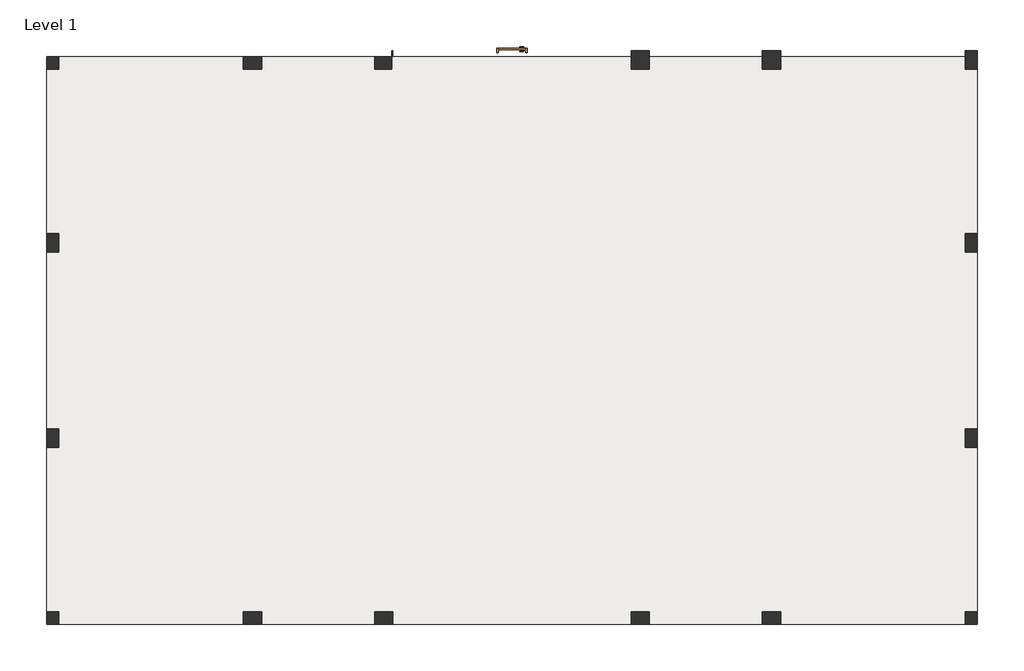
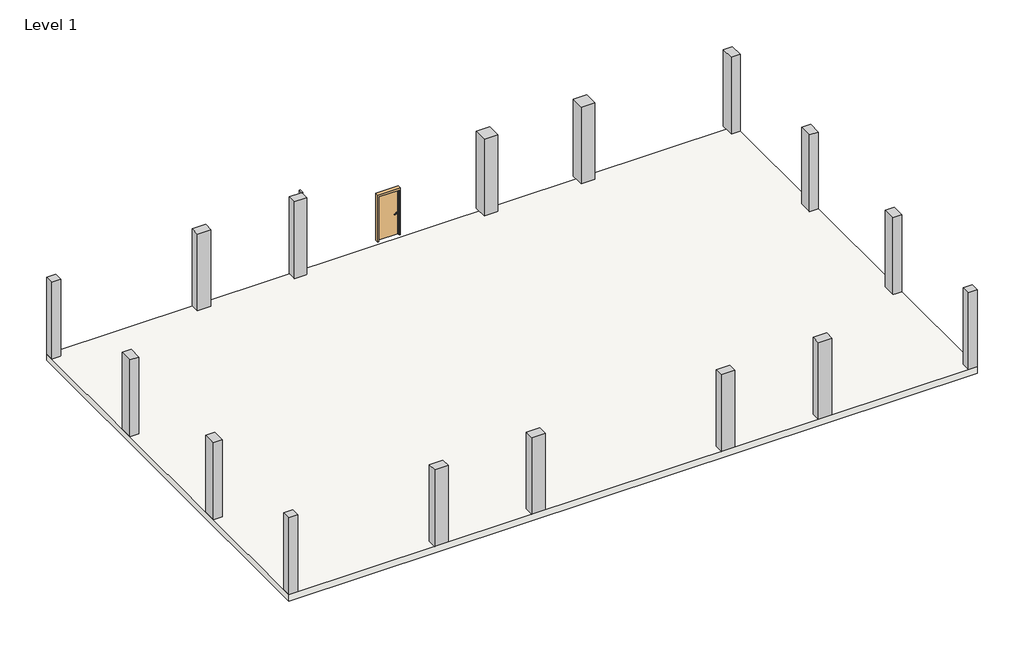
# One storey: 16 columns, 1 door, 1 slab.
"""IFC4 building model written with IfcOpenShell, lengths in millimetres."""

import ifcopenshell
import ifcopenshell.guid

model = None  # the IFC model being written
_history = None  # IfcOwnerHistory: only IFC2X3 demands one
_inside = {}  # id of a spatial element -> (the spatial element, [elements in it])
_under = {}  # id of a project, library or spatial element -> (it, [spatial elements below it])
_declared = {}  # id of a project -> (the project, [libraries it declares])
_typed = {}  # id of a type object -> (the type object, [elements of that type])
_made_of = {}  # id of a material, layer set ... -> (it, [elements and type objects made of it])


def new_model(schema):
    """Start an empty IFC model of exactly this schema.

    Asked for "IFC4X3", IfcOpenShell would pick the latest addendum, in which some entities
    have other attributes; the version numbers below select the first issue.
    IFC2X3 requires an IfcOwnerHistory on every rooted entity: one is made here for all.
    """
    global model, _history
    if schema == "IFC4X3":
        model = ifcopenshell.file(schema_version=(4, 3, 0, 0))
    else:
        model = ifcopenshell.file(schema=schema)
    _inside.clear()
    _under.clear()
    _declared.clear()
    _typed.clear()
    _made_of.clear()
    _history = None
    if model.schema == "IFC2X3":
        org = make("IfcOrganization", Name="unknown")
        user = make(
            "IfcPersonAndOrganization",
            ThePerson=make("IfcPerson", FamilyName="unknown"),
            TheOrganization=org,
        )
        app = make(
            "IfcApplication",
            ApplicationDeveloper=org,
            Version="unknown",
            ApplicationFullName="unknown",
            ApplicationIdentifier="unknown",
        )
        _history = make(
            "IfcOwnerHistory",
            OwningUser=user,
            OwningApplication=app,
            ChangeAction="ADDED",
            CreationDate=0,
        )
    return model


def make(cls, **values):
    """One entity of the class cls with the attributes given. An attribute that is None is left unset."""
    return model.create_entity(
        cls, **{name: value for name, value in values.items() if value is not None}
    )


def rooted(cls, **values):
    """An entity with a GlobalId (a new one), such as an element, a storey or a relation."""
    return make(cls, GlobalId=ifcopenshell.guid.new(), OwnerHistory=_history, **values)


def si_unit(unit_type, name, prefix=None):
    """IfcSIUnit, for example si_unit("LENGTHUNIT", "METRE", prefix="MILLI")."""
    return make("IfcSIUnit", UnitType=unit_type, Prefix=prefix, Name=name)


def assignment(units):
    """IfcUnitAssignment: the units of a project."""
    return None if units is None else make("IfcUnitAssignment", Units=units)


def point(xyz):
    """IfcCartesianPoint."""
    return None if xyz is None else make("IfcCartesianPoint", Coordinates=xyz)


def direction(xyz):
    """IfcDirection."""
    return None if xyz is None else make("IfcDirection", DirectionRatios=xyz)


def frame(location, z_axis=None, x_axis=None):
    """IfcAxis2Placement3D, a coordinate frame: its origin and axes. An axis left out is left unset."""
    return make(
        "IfcAxis2Placement3D",
        Location=point(location),
        Axis=direction(z_axis),
        RefDirection=direction(x_axis),
    )


def frame_2d(location, x_axis=None):
    """IfcAxis2Placement2D, a coordinate frame in the plane: its origin and x axis."""
    return make(
        "IfcAxis2Placement2D", Location=point(location), RefDirection=direction(x_axis)
    )


def origin():
    """The frame at (0, 0, 0) with its axes left unset."""
    return frame((0.0, 0.0, 0.0))


def origin_with_axes():
    """The frame at (0, 0, 0) with the z axis (0, 0, 1) and the x axis (1, 0, 0) written out."""
    return frame((0.0, 0.0, 0.0), z_axis=(0.0, 0.0, 1.0), x_axis=(1.0, 0.0, 0.0))


def place(relative_to, where):
    """IfcLocalPlacement: puts the frame where relative to a parent placement (None: the world)."""
    return make(
        "IfcLocalPlacement", PlacementRelTo=relative_to, RelativePlacement=where
    )


def context(
    kind, dimensions, precision=None, world=None, true_north=None, identifier=None
):
    """IfcGeometricRepresentationContext, for example the 3D "Model" context."""
    return make(
        "IfcGeometricRepresentationContext",
        ContextIdentifier=identifier,
        ContextType=kind,
        CoordinateSpaceDimension=dimensions,
        Precision=precision,
        WorldCoordinateSystem=world,
        TrueNorth=true_north,
    )


def project(units=None, contexts=None):
    """IfcProject with its units and contexts."""
    return rooted(
        "IfcProject",
        Name="project",
        RepresentationContexts=contexts,
        UnitsInContext=assignment(units),
    )


def spatial(cls, under=None, at=None, **own):
    """A site, building, storey or space (cls), placed at a placement, below another one or the project."""
    s = rooted(cls, ObjectPlacement=at, **own)
    if under is not None:
        _under.setdefault(under.id(), (under, []))[1].append(s)
    return s


def polyline(points):
    """IfcPolyline through the points."""
    return make("IfcPolyline", Points=[point(p) for p in points])


def circle_curve(where, radius):
    """IfcCircle in the frame where."""
    return make("IfcCircle", Position=where, Radius=radius)


def ellipse_curve(where, semi_axis1, semi_axis2):
    """IfcEllipse in the frame where."""
    return make(
        "IfcEllipse", Position=where, SemiAxis1=semi_axis1, SemiAxis2=semi_axis2
    )


def trimmed(basis, trim1, trim2, sense, master):
    """IfcTrimmedCurve: the piece of a basis curve between two trims."""
    return make(
        "IfcTrimmedCurve",
        BasisCurve=basis,
        Trim1=trim1,
        Trim2=trim2,
        SenseAgreement=sense,
        MasterRepresentation=master,
    )


def segment(curve, same_sense, transition):
    """IfcCompositeCurveSegment."""
    return make(
        "IfcCompositeCurveSegment",
        Transition=transition,
        SameSense=same_sense,
        ParentCurve=curve,
    )


def composite_curve(segments, self_intersect=None):
    """IfcCompositeCurve: segments joined end to end."""
    return make("IfcCompositeCurve", Segments=segments, SelfIntersect=self_intersect)


def outline(outer, holes=None, kind="AREA"):
    """IfcArbitraryClosedProfileDef: a profile drawn as a closed curve; with holes, ...WithVoids."""
    if holes is None:
        return make("IfcArbitraryClosedProfileDef", ProfileType=kind, OuterCurve=outer)
    return make(
        "IfcArbitraryProfileDefWithVoids",
        ProfileType=kind,
        OuterCurve=outer,
        InnerCurves=holes,
    )


def extrude(swept, where, along, depth):
    """IfcExtrudedAreaSolid: the profile swept, set in the frame where, extruded along a direction by depth."""
    return make(
        "IfcExtrudedAreaSolid",
        SweptArea=swept,
        Position=where,
        ExtrudedDirection=direction(along),
        Depth=depth,
    )


def faces_of(points, faces, orient=None, outer=None):
    """IfcFace entities. A face is a list of loops; a loop is a list of indices into points, from 0.

    orient and outer hold one flag for each loop. By default every Orientation is true, the
    first loop of a face is its IfcFaceOuterBound and the others are IfcFaceBound.
    """
    made = []
    for i, loops in enumerate(faces):
        bounds = []
        for j, loop in enumerate(loops):
            is_outer = j == 0 if outer is None else outer[i][j]
            bounds.append(
                make(
                    "IfcFaceOuterBound" if is_outer else "IfcFaceBound",
                    Bound=make("IfcPolyLoop", Polygon=[points[k] for k in loop]),
                    Orientation=True if orient is None else orient[i][j],
                )
            )
        made.append(make("IfcFace", Bounds=bounds))
    return made


def faceted_brep(points, faces, orient=None, outer=None, voids=None):
    """IfcFacetedBrep: a solid bounded by flat faces; with voids (closed shells), ...WithVoids."""
    shared = [point(p) for p in points]
    hull = make("IfcClosedShell", CfsFaces=faces_of(shared, faces, orient, outer))
    if voids is None:
        return make("IfcFacetedBrep", Outer=hull)
    return make(
        "IfcFacetedBrepWithVoids",
        Outer=hull,
        Voids=[
            make(cls, CfsFaces=faces_of(shared, fs, o, b)) for cls, fs, o, b in voids
        ],
    )


def shape(context_of_items, identifier, shape_type, items):
    """IfcShapeRepresentation: the items that make up one representation, for example the "Body"."""
    return make(
        "IfcShapeRepresentation",
        ContextOfItems=context_of_items,
        RepresentationIdentifier=identifier,
        RepresentationType=shape_type,
        Items=items,
    )


def source(mapping_origin, context_of_items, identifier, shape_type, items):
    """IfcRepresentationMap: a shape defined once, which mapped items show again and again."""
    return make(
        "IfcRepresentationMap",
        MappingOrigin=mapping_origin,
        MappedRepresentation=shape(context_of_items, identifier, shape_type, items),
    )


def transform(
    local_origin,
    x_axis=None,
    y_axis=None,
    z_axis=None,
    scale=None,
    scale2=None,
    scale3=None,
    uniform=True,
):
    """IfcCartesianTransformationOperator3D, or its non-uniform kind. x_axis, y_axis, z_axis: its Axis1, 2, 3."""
    if uniform:
        return make(
            "IfcCartesianTransformationOperator3D",
            Axis1=direction(x_axis),
            Axis2=direction(y_axis),
            LocalOrigin=point(local_origin),
            Scale=scale,
            Axis3=direction(z_axis),
        )
    return make(
        "IfcCartesianTransformationOperator3DnonUniform",
        Axis1=direction(x_axis),
        Axis2=direction(y_axis),
        LocalOrigin=point(local_origin),
        Scale=scale,
        Axis3=direction(z_axis),
        Scale2=scale2,
        Scale3=scale3,
    )


def mapped(mapping_source, mapping_target):
    """IfcMappedItem: shows the shape of a source again, moved by a transform."""
    return make(
        "IfcMappedItem", MappingSource=mapping_source, MappingTarget=mapping_target
    )


def made_of(thing, what):
    """Note that an element or type object is made of a material, layer set ...; save() writes the relation."""
    if what is not None:
        _made_of.setdefault(what.id(), (what, []))[1].append(thing)
    return thing


def element(
    cls,
    number,
    at=None,
    inside=None,
    cuts=None,
    type_object=None,
    material=None,
    context=None,
    identifier="Body",
    shape_type=None,
    held_by="IfcProductDefinitionShape",
    body=None,
    shapes=None,
    **own,
):
    """One element of the class cls, such as IfcWall. Its Tag is "e" and its number.

    at: its placement. inside: the storey or other place that contains it. cuts: it is an
    opening in that element (IfcRelVoidsElement). A single representation is given by context,
    identifier, shape_type and body (its items); several are given by shapes. held_by: the class
    of the entity that holds the representations. save() writes the other relations.
    """
    e = rooted(cls, Tag="e%d" % number, ObjectPlacement=at, **own)
    if body is not None:
        shapes = [shape(context, identifier, shape_type, body)]
    if shapes is not None:
        e.Representation = make(held_by, Representations=shapes)
    if inside is not None:
        _inside.setdefault(inside.id(), (inside, []))[1].append(e)
    if cuts is not None:
        rooted(
            "IfcRelVoidsElement", RelatingBuildingElement=cuts, RelatedOpeningElement=e
        )
    if type_object is not None:
        _typed.setdefault(type_object.id(), (type_object, []))[1].append(e)
    return made_of(e, material)


def aggregate(whole, parts):
    """IfcRelAggregates: a whole, such as a stair, and the parts it consists of."""
    return rooted("IfcRelAggregates", RelatingObject=whole, RelatedObjects=parts)


def save(model, path):
    """Write the relations noted so far, then the file.

    IfcRelAggregates (storeys below a building ...), IfcRelContainedInSpatialStructure (elements
    in a storey), IfcRelDefinesByType, IfcRelAssociatesMaterial and IfcRelDeclares: one each for
    every whole, place, type object, material and project.
    """
    for whole, parts in _under.values():
        aggregate(whole, parts)
    for where, things in _inside.values():
        rooted(
            "IfcRelContainedInSpatialStructure",
            RelatedElements=things,
            RelatingStructure=where,
        )
    for kind, things in _typed.values():
        rooted("IfcRelDefinesByType", RelatedObjects=things, RelatingType=kind)
    for what, things in _made_of.values():
        rooted("IfcRelAssociatesMaterial", RelatedObjects=things, RelatingMaterial=what)
    for by, libraries in _declared.values():
        rooted("IfcRelDeclares", RelatingContext=by, RelatedDefinitions=libraries)
    model.write(path)


def plane_surface(at):
    """IfcPlane: the flat surface through the origin of the frame at, square to its z axis."""
    return make("IfcPlane", Position=at)


def cylinder_surface(at, radius):
    """IfcCylindricalSurface: all points at the distance radius from the z axis of the frame at."""
    return make("IfcCylindricalSurface", Position=at, Radius=radius)


def revolved_surface(curve, axis_point, axis_direction):
    """IfcSurfaceOfRevolution: the curve turned about the line through axis_point along axis_direction."""
    return make(
        "IfcSurfaceOfRevolution",
        SweptCurve=make("IfcArbitraryOpenProfileDef", ProfileType="CURVE", Curve=curve),
        AxisPosition=make("IfcAxis1Placement", Location=point(axis_point), Axis=direction(axis_direction)),
    )


def advanced_brep(points, edges, surfaces, faces):
    """IfcAdvancedBrep: a solid bounded by faces that lie on surfaces and meet in shared edges.

    An edge is (start, end): straight between two places in points (the first is 0);
    or (start, end, curve); or (start, end, curve, False) where it runs against its curve.
    A face is (place in surfaces, loops), or (place, loops, False) where it looks against
    its surface's normal. A loop lists edges by number (the first is 1), with a minus sign
    where the edge is run from its end to its start. The first loop is the outer one.
    """
    corners = [point(p) for p in points]
    vertices = [make("IfcVertexPoint", VertexGeometry=c) for c in corners]
    made = []
    for start, end, *more in edges:
        made.append(
            make(
                "IfcEdgeCurve",
                EdgeStart=vertices[start],
                EdgeEnd=vertices[end],
                EdgeGeometry=more[0] if more else make("IfcPolyline", Points=[corners[start], corners[end]]),
                SameSense=more[1] if len(more) > 1 else True,
            )
        )
    hull = []
    for where, loops, *sense in faces:
        bounds = []
        for j, loop in enumerate(loops):
            ring = [make("IfcOrientedEdge", EdgeElement=made[abs(k) - 1], Orientation=k > 0) for k in loop]
            bounds.append(
                make(
                    "IfcFaceOuterBound" if j == 0 else "IfcFaceBound",
                    Bound=make("IfcEdgeLoop", EdgeList=ring),
                    Orientation=True,
                )
            )
        hull.append(make("IfcAdvancedFace", Bounds=bounds, FaceSurface=surfaces[where], SameSense=sense[0] if sense else True))
    return make("IfcAdvancedBrep", Outer=make("IfcClosedShell", CfsFaces=hull))


def door_58febf71(model_context):
    return source(origin(), model_context, "Body", "SolidModel", [
        advanced_brep(
        [(-392.190625, -76.1375, 1016.0), (-372.190625, -76.1375, 1016.0), (-392.190625, -46.1375, 1016.0), (-372.190625, -46.1375, 1016.0), (-367.190625, -41.1375, 1016.0), (-367.190625, -21.1375, 1016.0), (-262.190625, -21.1375, 1016.0), (-262.190625, -41.1375, 1016.0)],
        [
            (0, 1, circle_curve(frame((-382.190625, -76.1375, 1016.0), z_axis=(0.0, -1.0, 0.0), x_axis=(1.0, 0.0, 0.0)), 10.0)),
            (1, 0, circle_curve(frame((-382.190625, -76.1375, 1016.0), z_axis=(0.0, -1.0, 0.0), x_axis=(1.0, 0.0, 0.0)), 10.0)),
            (0, 2),
            (2, 3, circle_curve(frame((-382.190625, -46.1375, 1016.0), z_axis=(0.0, -1.0, 0.0), x_axis=(1.0, 0.0, 0.0)), 10.0)),
            (3, 1),
            (3, 2, circle_curve(frame((-382.190625, -46.1375, 1016.0), z_axis=(0.0, -1.0, 0.0), x_axis=(1.0, 0.0, 0.0)), 10.0)),
            (4, 3, circle_curve(frame((-367.190625, -46.1375, 1016.0), z_axis=(0.0, 0.0, 1.0), x_axis=(-1.0, 0.0, 0.0)), 5.0)),
            (2, 5, circle_curve(frame((-367.190625, -46.1375, 1016.0), z_axis=(0.0, 0.0, -1.0), x_axis=(-1.0, 0.0, 0.0)), 25.0)),
            (5, 4, circle_curve(frame((-367.190625, -31.1375, 1016.0), z_axis=(-1.0, 0.0, 0.0), x_axis=(0.0, -1.0, 0.0)), 10.0)),
            (4, 5, circle_curve(frame((-367.190625, -31.1375, 1016.0), z_axis=(-1.0, 0.0, 0.0), x_axis=(0.0, -1.0, 0.0)), 10.0)),
            (6, 7, circle_curve(frame((-262.190625, -31.1375, 1016.0), z_axis=(1.0, 0.0, 0.0), x_axis=(0.0, -1.0, 0.0)), 10.0)),
            (7, 6, circle_curve(frame((-262.190625, -31.1375, 1016.0), z_axis=(1.0, 0.0, 0.0), x_axis=(0.0, -1.0, 0.0)), 10.0)),
            (5, 6),
            (7, 4),
        ],
        [
            plane_surface(frame((-382.190625, -76.1375, 1016.0), z_axis=(0.0, -1.0, 0.0), x_axis=(0.0, 0.0, 1.0))),
            cylinder_surface(frame((-382.190625, -76.1375, 1016.0), z_axis=(0.0, -1.0, 0.0), x_axis=(1.0, 0.0, 0.0)), 10.0),
            revolved_surface(trimmed(ellipse_curve(frame((-382.190625, -46.1375, 1016.0), z_axis=(0.0, -1.0, 0.0), x_axis=(1.0, 0.0, 0.0)), 10.0, 10.0), [point((-392.190625, -46.1375, 1016.0))], [point((-372.190625, -46.1375, 1016.0))], True, "CARTESIAN"), (-367.190625, -46.1375, 1016.0), (0.0, 0.0, -1.0)),
            revolved_surface(trimmed(ellipse_curve(frame((-382.190625, -46.1375, 1016.0), z_axis=(0.0, -1.0, 0.0), x_axis=(1.0, 0.0, 0.0)), 10.0, 10.0), [point((-372.190625, -46.1375, 1016.0))], [point((-392.190625, -46.1375, 1016.0))], True, "CARTESIAN"), (-367.190625, -46.1375, 1016.0), (0.0, 0.0, -1.0)),
            plane_surface(frame((-262.190625, -31.1375, 1016.0), z_axis=(1.0, 0.0, 0.0), x_axis=(0.0, 0.0, 1.0))),
            cylinder_surface(frame((-367.190625, -31.1375, 1016.0), z_axis=(-1.0, 0.0, 0.0), x_axis=(0.0, -1.0, 0.0)), 10.0),
        ],
        [
            (0, [[1, 2]]),
            (1, [[-1, 3, 4, 5]]),
            (1, [[-2, -5, 6, -3]]),
            (2, [[7, -4, 8, 9]]),
            (3, [[-8, -6, -7, 10]]),
            (4, [[11, 12]]),
            (5, [[-9, 13, -12, 14]]),
            (5, [[-10, -14, -11, -13]]),
        ],
    ),
        extrude(outline(composite_curve([segment(trimmed(circle_curve(frame_2d((1016.0, -384.690625)), 30.0), [point((1016.0, -414.690625))], [point((1016.0, -354.690625))], False, "CARTESIAN"), True, "CONTINUOUS"), segment(trimmed(circle_curve(frame_2d((1016.0, -384.690625)), 30.0), [point((1016.0, -354.690625))], [point((1016.0, -414.690625))], False, "CARTESIAN"), True, "CONTINUOUS")], self_intersect=False)), frame((0.0, -84.1375, 0.0), z_axis=(0.0, 1.0, 0.0), x_axis=(0.0, 0.0, 1.0)), (0.0, 0.0, 1.0), 8.0),
        advanced_brep(
        [(-392.190625, -136.5875, 1016.0), (-372.190625, -136.5875, 1016.0), (-372.190625, -166.5875, 1016.0), (-392.190625, -166.5875, 1016.0), (-367.190625, -171.5875, 1016.0), (-367.190625, -191.5875, 1016.0), (-262.190625, -191.5875, 1016.0), (-262.190625, -171.5875, 1016.0)],
        [
            (0, 1, circle_curve(frame((-382.190625, -136.5875, 1016.0), z_axis=(0.0, 1.0, 0.0), x_axis=(1.0, 0.0, 0.0)), 10.0)),
            (1, 0, circle_curve(frame((-382.190625, -136.5875, 1016.0), z_axis=(0.0, 1.0, 0.0), x_axis=(1.0, 0.0, 0.0)), 10.0)),
            (1, 2),
            (2, 3, circle_curve(frame((-382.190625, -166.5875, 1016.0), z_axis=(0.0, 1.0, 0.0), x_axis=(1.0, 0.0, 0.0)), 10.0)),
            (3, 0),
            (3, 2, circle_curve(frame((-382.190625, -166.5875, 1016.0), z_axis=(0.0, 1.0, 0.0), x_axis=(1.0, 0.0, 0.0)), 10.0)),
            (4, 5, circle_curve(frame((-367.190625, -181.5875, 1016.0), z_axis=(-1.0, 0.0, 0.0), x_axis=(0.0, 1.0, 0.0)), 10.0)),
            (5, 3, circle_curve(frame((-367.190625, -166.5875, 1016.0), z_axis=(0.0, 0.0, -1.0), x_axis=(-1.0, 0.0, 0.0)), 25.0)),
            (2, 4, circle_curve(frame((-367.190625, -166.5875, 1016.0), z_axis=(0.0, 0.0, 1.0), x_axis=(-1.0, 0.0, 0.0)), 5.0)),
            (5, 4, circle_curve(frame((-367.190625, -181.5875, 1016.0), z_axis=(-1.0, 0.0, 0.0), x_axis=(0.0, 1.0, 0.0)), 10.0)),
            (6, 7, circle_curve(frame((-262.190625, -181.5875, 1016.0), z_axis=(1.0, 0.0, 0.0), x_axis=(0.0, 1.0, 0.0)), 10.0)),
            (7, 6, circle_curve(frame((-262.190625, -181.5875, 1016.0), z_axis=(1.0, 0.0, 0.0), x_axis=(0.0, 1.0, 0.0)), 10.0)),
            (4, 7),
            (6, 5),
        ],
        [
            plane_surface(frame((-382.190625, -136.5875, 1016.0), z_axis=(0.0, 1.0, 0.0), x_axis=(0.0, 0.0, 1.0))),
            cylinder_surface(frame((-382.190625, -136.5875, 1016.0), z_axis=(0.0, 1.0, 0.0), x_axis=(1.0, 0.0, 0.0)), 10.0),
            revolved_surface(trimmed(ellipse_curve(frame((-382.190625, -166.5875, 1016.0), z_axis=(0.0, -1.0, 0.0), x_axis=(1.0, 0.0, 0.0)), 10.0, 10.0), [point((-392.190625, -166.5875, 1016.0))], [point((-372.190625, -166.5875, 1016.0))], True, "CARTESIAN"), (-367.190625, -166.5875, 1016.0), (0.0, 0.0, -1.0)),
            revolved_surface(trimmed(ellipse_curve(frame((-382.190625, -166.5875, 1016.0), z_axis=(0.0, -1.0, 0.0), x_axis=(1.0, 0.0, 0.0)), 10.0, 10.0), [point((-372.190625, -166.5875, 1016.0))], [point((-392.190625, -166.5875, 1016.0))], True, "CARTESIAN"), (-367.190625, -166.5875, 1016.0), (0.0, 0.0, -1.0)),
            plane_surface(frame((-262.190625, -181.5875, 1016.0), z_axis=(1.0, 0.0, 0.0), x_axis=(0.0, 0.0, 1.0))),
            cylinder_surface(frame((-367.190625, -181.5875, 1016.0), z_axis=(-1.0, 0.0, 0.0), x_axis=(0.0, 1.0, 0.0)), 10.0),
        ],
        [
            (0, [[1, 2]]),
            (1, [[3, 4, 5, -2]]),
            (1, [[-5, 6, -3, -1]]),
            (2, [[7, 8, -4, 9]]),
            (3, [[10, -9, -6, -8]]),
            (4, [[11, 12]]),
            (5, [[13, -11, 14, -7]]),
            (5, [[-14, -12, -13, -10]]),
        ],
    ),
        extrude(outline(composite_curve([segment(trimmed(circle_curve(frame_2d((1016.0, -384.690625)), 30.0), [point((1016.0, -414.690625))], [point((1016.0, -354.690625))], False, "CARTESIAN"), True, "CONTINUOUS"), segment(trimmed(circle_curve(frame_2d((1016.0, -384.690625)), 30.0), [point((1016.0, -354.690625))], [point((1016.0, -414.690625))], False, "CARTESIAN"), True, "CONTINUOUS")], self_intersect=False)), frame((0.0, -136.5875, 0.0), z_axis=(0.0, 1.0, 0.0), x_axis=(0.0, 0.0, 1.0)), (0.0, 0.0, 1.0), 8.0),
        faceted_brep([(457.2, -79.375, 0.0), (441.325, -79.375, 0.0), (441.325, -31.75, 0.0), (457.2, -31.75, 0.0), (457.2, 17.4625, 0.0), (508.0, 17.4625, 0.0), (508.0, -128.5875, 0.0), (457.2, -128.5875, 0.0), (457.2, -128.5875, 2133.6), (457.2, -79.375, 2133.6), (508.0, -128.5875, 2235.2), (-508.0, -128.5875, 2235.2), (-508.0, -128.5875, 0.0), (-457.2, -128.5875, 0.0), (-457.2, -128.5875, 2133.6), (508.0, 17.4625, 2235.2), (457.2, 17.4625, 2133.6), (-457.2, 17.4625, 2133.6), (-457.2, 17.4625, 0.0), (-508.0, 17.4625, 0.0), (-508.0, 17.4625, 2235.2), (457.2, -31.75, 2133.6), (441.325, -31.75, 2117.725), (-441.325, -31.75, 2117.725), (-441.325, -31.75, 0.0), (-457.2, -31.75, 0.0), (-457.2, -31.75, 2133.6), (441.325, -79.375, 2117.725), (-457.2, -79.375, 2133.6), (-457.2, -79.375, 0.0), (-441.325, -79.375, 0.0), (-441.325, -79.375, 2117.725)], [[[0, 1, 2, 3, 4, 5, 6, 7]], [[7, 8, 9, 0]], [[6, 10, 11, 12, 13, 14, 8, 7]], [[5, 15, 10, 6]], [[4, 16, 17, 18, 19, 20, 15, 5]], [[3, 21, 16, 4]], [[2, 22, 23, 24, 25, 26, 21, 3]], [[1, 27, 22, 2]], [[0, 9, 28, 29, 30, 31, 27, 1]], [[8, 14, 28, 9]], [[16, 21, 26, 17]], [[22, 27, 31, 23]], [[12, 19, 18, 25, 24, 30, 29, 13]], [[13, 29, 28, 14]], [[11, 20, 19, 12]], [[17, 26, 25, 18]], [[23, 31, 30, 24]], [[15, 20, 11, 10]]]),
        extrude(outline(polyline([(457.2, -84.1375), (457.2, -128.5875), (-457.2, -128.5875), (-457.2, -84.1375), (457.2, -84.1375)])), origin_with_axes(), (0.0, 0.0, 1.0), 2133.6),
    ])


model = new_model("IFC4")

# Units and contexts
model_context = context("Model", 3, world=origin())
ifc_project = project(units=[si_unit("LENGTHUNIT", "METRE", prefix="MILLI")], contexts=[model_context])

# Site, building, storey
site = spatial("IfcSite", under=ifc_project)
building = spatial("IfcBuilding", under=site)
storey = spatial("IfcBuildingStorey", under=building, Name="Level 1", Elevation=0.0)

# Columns
placement = place(None, origin())
element("IfcColumn", 1, ObjectType="Rectangular Column : 24\" x 24\"", at=placement, inside=storey, context=model_context, shape_type="SweptSolid", body=[
    extrude(outline(polyline([(-16253.4122732, 9291.5015304), (-16253.4122732, 8885.1015304), (-16659.8122732, 8885.1015304), (-16659.8122732, 9291.5015304), (-16253.4122732, 9291.5015304)])), origin_with_axes(), (0.0, 0.0, 1.0), 3657.6),
])
element("IfcColumn", 2, ObjectType="Rectangular Column : 24\" x 24\"", at=placement, inside=storey, context=model_context, shape_type="SweptSolid", body=[
    extrude(outline(polyline([(-16253.4122732, 3398.7015304), (-16253.4122732, 2789.1015304), (-16659.8122732, 2789.1015304), (-16659.8122732, 3398.7015304), (-16253.4122732, 3398.7015304)])), origin_with_axes(), (0.0, 0.0, 1.0), 3657.6),
])
element("IfcColumn", 3, ObjectType="Rectangular Column : 24\" x 24\"", at=placement, inside=storey, context=model_context, shape_type="SweptSolid", body=[
    extrude(outline(polyline([(-9497.0122732, 8885.1015304), (-10106.6122732, 8885.1015304), (-10106.6122732, 9291.5015304), (-9497.0122732, 9291.5015304), (-9497.0122732, 8885.1015304)])), origin_with_axes(), (0.0, 0.0, 1.0), 3657.6),
])
element("IfcColumn", 4, ObjectType="Rectangular Column : 24\" x 24\"", at=placement, inside=storey, context=model_context, shape_type="SweptSolid", body=[
    extrude(outline(polyline([(-5174.2497732, 9494.7015304), (-5128.2122732, 9494.7015304), (-5128.2122732, 9301.0265304), (-5174.2497732, 9301.0265304), (-5174.2497732, 9494.7015304)])), origin_with_axes(), (0.0, 0.0, 1.0), 3657.6),
    extrude(outline(polyline([(-5737.8122732, 8885.1015304), (-5737.8122732, 9291.5015304), (-5174.2497732, 9291.5015304), (-5174.2497732, 8885.1015304), (-5737.8122732, 8885.1015304)])), origin_with_axes(), (0.0, 0.0, 1.0), 3657.6),
])
element("IfcColumn", 5, ObjectType="Rectangular Column : 24\" x 24\"", at=placement, inside=storey, context=model_context, shape_type="SweptSolid", body=[
    extrude(outline(polyline([(3406.1877268, 9494.7015304), (3406.1877268, 8885.1015304), (2796.5877268, 8885.1015304), (2796.5877268, 9494.7015304), (3406.1877268, 9494.7015304)])), origin_with_axes(), (0.0, 0.0, 1.0), 3657.6),
])
element("IfcColumn", 6, ObjectType="Rectangular Column : 24\" x 24\"", at=placement, inside=storey, context=model_context, shape_type="SweptSolid", body=[
    extrude(outline(polyline([(7774.9877268, 9494.7015304), (7774.9877268, 8885.1015304), (7165.3877268, 8885.1015304), (7165.3877268, 9494.7015304), (7774.9877268, 9494.7015304)])), origin_with_axes(), (0.0, 0.0, 1.0), 3657.6),
])
element("IfcColumn", 7, ObjectType="Rectangular Column : 24\" x 24\"", at=placement, inside=storey, context=model_context, shape_type="SweptSolid", body=[
    extrude(outline(polyline([(13921.7877268, 8885.1015304), (13921.7877268, 9494.7015304), (14328.1877268, 9494.7015304), (14328.1877268, 8885.1015304), (13921.7877268, 8885.1015304)])), origin_with_axes(), (0.0, 0.0, 1.0), 3657.6),
])
element("IfcColumn", 8, ObjectType="Rectangular Column : 24\" x 24\"", at=placement, inside=storey, context=model_context, shape_type="SweptSolid", body=[
    extrude(outline(polyline([(13921.7877268, 2789.1015304), (13921.7877268, 3398.7015304), (14328.1877268, 3398.7015304), (14328.1877268, 2789.1015304), (13921.7877268, 2789.1015304)])), origin_with_axes(), (0.0, 0.0, 1.0), 3657.6),
])
element("IfcColumn", 9, ObjectType="Rectangular Column : 24\" x 24\"", at=placement, inside=storey, context=model_context, shape_type="SweptSolid", body=[
    extrude(outline(polyline([(13921.7877268, -3713.2984696), (13921.7877268, -3103.6984696), (14328.1877268, -3103.6984696), (14328.1877268, -3713.2984696), (13921.7877268, -3713.2984696)])), origin_with_axes(), (0.0, 0.0, 1.0), 3657.6),
])
element("IfcColumn", 10, ObjectType="Rectangular Column : 24\" x 24\"", at=placement, inside=storey, context=model_context, shape_type="SweptSolid", body=[
    extrude(outline(polyline([(13921.7877268, -9606.0984696), (13921.7877268, -9199.6984696), (14328.1877268, -9199.6984696), (14328.1877268, -9606.0984696), (13921.7877268, -9606.0984696)])), origin_with_axes(), (0.0, 0.0, 1.0), 3657.6),
])
element("IfcColumn", 11, ObjectType="Rectangular Column : 24\" x 24\"", at=placement, inside=storey, context=model_context, shape_type="SweptSolid", body=[
    extrude(outline(polyline([(7165.3877268, -9199.6984696), (7774.9877268, -9199.6984696), (7774.9877268, -9606.0984696), (7165.3877268, -9606.0984696), (7165.3877268, -9199.6984696)])), origin_with_axes(), (0.0, 0.0, 1.0), 3657.6),
])
element("IfcColumn", 12, ObjectType="Rectangular Column : 24\" x 24\"", at=placement, inside=storey, context=model_context, shape_type="SweptSolid", body=[
    extrude(outline(polyline([(2796.5877268, -9199.6984696), (3406.1877268, -9199.6984696), (3406.1877268, -9606.0984696), (2796.5877268, -9606.0984696), (2796.5877268, -9199.6984696)])), origin_with_axes(), (0.0, 0.0, 1.0), 3657.6),
])
element("IfcColumn", 13, ObjectType="Rectangular Column : 24\" x 24\"", at=placement, inside=storey, context=model_context, shape_type="SweptSolid", body=[
    extrude(outline(polyline([(-5737.8122732, -9199.6984696), (-5128.2122732, -9199.6984696), (-5128.2122732, -9606.0984696), (-5737.8122732, -9606.0984696), (-5737.8122732, -9199.6984696)])), origin_with_axes(), (0.0, 0.0, 1.0), 3657.6),
])
element("IfcColumn", 14, ObjectType="Rectangular Column : 24\" x 24\"", at=placement, inside=storey, context=model_context, shape_type="SweptSolid", body=[
    extrude(outline(polyline([(-10106.6122732, -9199.6984696), (-9497.0122732, -9199.6984696), (-9497.0122732, -9606.0984696), (-10106.6122732, -9606.0984696), (-10106.6122732, -9199.6984696)])), origin_with_axes(), (0.0, 0.0, 1.0), 3657.6),
])
element("IfcColumn", 15, ObjectType="Rectangular Column : 24\" x 24\"", at=placement, inside=storey, context=model_context, shape_type="SweptSolid", body=[
    extrude(outline(polyline([(-16659.8122732, -9199.6984696), (-16253.4122732, -9199.6984696), (-16253.4122732, -9606.0984696), (-16659.8122732, -9606.0984696), (-16659.8122732, -9199.6984696)])), origin_with_axes(), (0.0, 0.0, 1.0), 3657.6),
])
element("IfcColumn", 16, ObjectType="Rectangular Column : 24\" x 24\"", at=placement, inside=storey, context=model_context, shape_type="SweptSolid", body=[
    extrude(outline(polyline([(-16253.4122732, -3103.6984696), (-16253.4122732, -3713.2984696), (-16659.8122732, -3713.2984696), (-16659.8122732, -3103.6984696), (-16253.4122732, -3103.6984696)])), origin_with_axes(), (0.0, 0.0, 1.0), 3657.6),
])

# Door
door_shape = door_58febf71(model_context)
element("IfcDoor", 17, ObjectType="Door-Passage-Single-Flush : 36\" x 84\"", at=placement, inside=storey, context=model_context, shape_type="MappedRepresentation", body=[
    mapped(door_shape, transform((-1165.8122732, 9442.3140304, 0.0), x_axis=(-1.0, 0.0, 0.0), y_axis=(0.0, -1.0, 0.0), z_axis=(0.0, 0.0, 1.0))),
])

# Slab
element("IfcSlab", 18, ObjectType="Generic - 12\"", at=placement, inside=storey, context=model_context, shape_type="SweptSolid", body=[
    extrude(outline(polyline([(-16659.8122732, 9291.5015304), (14328.1877268, 9291.5015304), (14328.1877268, -9606.0984696), (-16659.8122732, -9606.0984696), (-16659.8122732, 9291.5015304)])), frame((0.0, 0.0, -304.8), z_axis=(0.0, 0.0, 1.0), x_axis=(1.0, 0.0, 0.0)), (0.0, 0.0, 1.0), 304.8),
])

save(model, "model.ifc")

# Revit data of these elements
# Type "Rectangular Column : 24\" x 24\""
#   Assembly Code = "B1010200"
#   Depth = 2' - 0"
#   Offset Base = 0' - 0"
#   Offset Top = 0' - 0"
#   Width = 2' - 0"
#   Material = none
# Type "Door-Passage-Single-Flush : 36\" x 84\""
#   Type Mark = "1"
#   Assembly Code = "B2030200"
#   Analytic Construction = "Wooden"
#   Thickness = 0' - 1 3/4"
#   Thermal Resistance (R) = 2.5876 (h·ft²·°F)/BTU
#   Swing Angle [instance default] = 90.00°
#   Strike Height = 3' - 4"
#   Rough Width [instance default] = 3' - 4"
#   Rough Height [instance default] = 7' - 4"
#   MF Opening Height [instance default] = 0' - 4"
#   MF Opening Width [instance default] = 0' - 4"
#   Inset Calculate [instance default] = 0' - 4"
#   Masonry Inset [instance default] = 0' - 1"
#   Height = 7' - 0"
#   Width = 3' - 0"
#   Heat Transfer Coefficient (U) = 0.3865 BTU/(h·ft²·°F)
#   Masonry Frame Depth = 0' - 5 3/4"
#   Define Thermal Properties by = 1
#   Masonry Frame [instance default] = yes
#   Function = 1
#   Dry Wall Frame [instance default] = no
#   Panel Material = Wood - Birch
#   Frame Material = Metal - Paint Finish - Grey
#   Door Handle Material = Aluminum
#   Visual Light Transmittance = 0
#   Solar Heat Gain Coefficient = 0
#   Wall Closure = (empty or 0)
# Type "Generic - 12\""
#   Assembly Code = "B1010"
#   Function = 0
#   Layers, outside or top first: 1' - 0" no material (function 1)
# Elements 1, 2, 3, 4, 7, 8, 9, 10, 11, 12, 13, 14, 15, 16 (IfcColumn, "Rectangular Column : 24\" x 24\"")
#   Phase Created = New Construction
#   Materials on its faces: "Default Wall"
# Elements 5, 6 (IfcColumn, "Rectangular Column : 24\" x 24\"")
#   Phase Created = New Construction
# Element 17 (IfcDoor, "Door-Passage-Single-Flush : 36\" x 84\"")
#   Swing Angle = 90.00°
#   Rough Width = 3' - 4"
#   Rough Height = 7' - 4"
#   Masonry Inset = 0' - 1"
#   MF Opening Width = 0' - 4"
#   MF Opening Height = 0' - 4"
#   Inset Calculate = 0' - 4"
#   Masonry Frame = yes
#   Dry Wall Frame = no
#   Phase Created = New Construction
#   Materials on its faces: "Aluminum", "Metal - Paint Finish - Grey", "Wood - Birch"
# Element 18 (IfcSlab, "Generic - 12\"")
#   built-in parameter 1001955 = 1.5708 (stored number, unit not read)
#   Height Offset From Level = 0' - 0"
#   Phase Created = New Construction
#   Materials on its faces: "Default Floor"
# Materials
#   "Wood - Birch": class "Wood", colour RGB 166 116 52, transparency 0, Cost = 0
#   "Metal - Paint Finish - Grey": class "Paint", colour RGB 104 104 104, transparency 0, Cost = 0
#   "Aluminum": class "Metal", colour RGB 247 247 247, transparency 0, Description = "Aluminum 6061", Cost = 0
#   "Default Wall": class "Miscellaneous", colour RGB 128 128 128, transparency 0, Cost = 0
#   "Default Floor": class "Miscellaneous", colour RGB 128 128 128, transparency 0, Cost = 0
